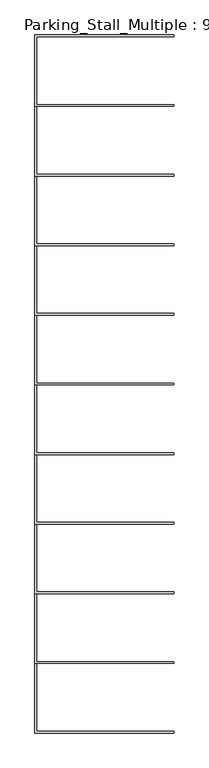
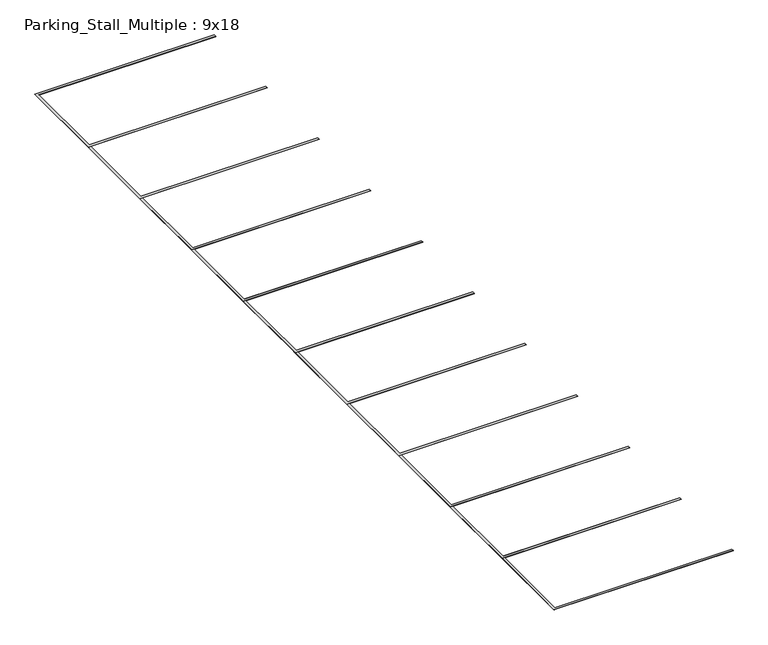
"""IFC4 building model written with IfcOpenShell, lengths in millimetres: proxy geometry, Parking_Stall_Multiple : 9x18."""

from ifc_helpers import new_model, si_unit, origin, origin_with_axes, place, context, project, spatial, polyline, outline, extrude, source, transform, mapped, element, save


def parking_stall_multiple_9x18_9482d3cf(model_context):
    return source(origin(), model_context, "Body", "SweptSolid", [
        extrude(outline(polyline([(5486.4, 24688.8), (0.0, 24688.8), (0.0, 27508.2), (5486.4, 27508.2), (5486.4, 27432.0), (76.2, 27432.0), (76.2, 24765.0), (5486.4, 24765.0), (5486.4, 24688.8)])), origin_with_axes(), (0.0, 0.0, 1.0), 6.35),
        extrude(outline(polyline([(5486.4, 21945.6), (0.0, 21945.6), (0.0, 24765.0), (5486.4, 24765.0), (5486.4, 24688.8), (76.2, 24688.8), (76.2, 22021.8), (5486.4, 22021.8), (5486.4, 21945.6)])), origin_with_axes(), (0.0, 0.0, 1.0), 6.35),
        extrude(outline(polyline([(5486.4, 19202.4), (0.0, 19202.4), (0.0, 22021.8), (5486.4, 22021.8), (5486.4, 21945.6), (76.2, 21945.6), (76.2, 19278.6), (5486.4, 19278.6), (5486.4, 19202.4)])), origin_with_axes(), (0.0, 0.0, 1.0), 6.35),
        extrude(outline(polyline([(5486.4, 16459.2), (0.0, 16459.2), (0.0, 19278.6), (5486.4, 19278.6), (5486.4, 19202.4), (76.2, 19202.4), (76.2, 16535.4), (5486.4, 16535.4), (5486.4, 16459.2)])), origin_with_axes(), (0.0, 0.0, 1.0), 6.35),
        extrude(outline(polyline([(5486.4, 13716.0), (0.0, 13716.0), (0.0, 16535.4), (5486.4, 16535.4), (5486.4, 16459.2), (76.2, 16459.2), (76.2, 13792.2), (5486.4, 13792.2), (5486.4, 13716.0)])), origin_with_axes(), (0.0, 0.0, 1.0), 6.35),
        extrude(outline(polyline([(5486.4, 10972.8), (0.0, 10972.8), (0.0, 13792.2), (5486.4, 13792.2), (5486.4, 13716.0), (76.2, 13716.0), (76.2, 11049.0), (5486.4, 11049.0), (5486.4, 10972.8)])), origin_with_axes(), (0.0, 0.0, 1.0), 6.35),
        extrude(outline(polyline([(5486.4, 8229.6), (0.0, 8229.6), (0.0, 11049.0), (5486.4, 11049.0), (5486.4, 10972.8), (76.2, 10972.8), (76.2, 8305.8), (5486.4, 8305.8), (5486.4, 8229.6)])), origin_with_axes(), (0.0, 0.0, 1.0), 6.35),
        extrude(outline(polyline([(5486.4, 5486.4), (0.0, 5486.4), (0.0, 8305.8), (5486.4, 8305.8), (5486.4, 8229.6), (76.2, 8229.6), (76.2, 5562.6), (5486.4, 5562.6), (5486.4, 5486.4)])), origin_with_axes(), (0.0, 0.0, 1.0), 6.35),
        extrude(outline(polyline([(5486.4, 2743.2), (0.0, 2743.2), (0.0, 5562.6), (5486.4, 5562.6), (5486.4, 5486.4), (76.2, 5486.4), (76.2, 2819.4), (5486.4, 2819.4), (5486.4, 2743.2)])), origin_with_axes(), (0.0, 0.0, 1.0), 6.35),
        extrude(outline(polyline([(5486.4, 0.0), (0.0, 0.0), (0.0, 2819.4), (5486.4, 2819.4), (5486.4, 2743.2), (76.2, 2743.2), (76.2, 76.2), (5486.4, 76.2), (5486.4, 0.0)])), origin_with_axes(), (0.0, 0.0, 1.0), 6.35),
    ])


if __name__ == "__main__":
    model = new_model("IFC4")
    model_context = context("Model", 3, world=origin())
    ifc_project = project(units=[si_unit("LENGTHUNIT", "METRE", prefix="MILLI")], contexts=[model_context])
    site = spatial("IfcSite", under=ifc_project)
    building = spatial("IfcBuilding", under=site)
    placement = place(None, origin())
    parking_stall_multiple_9x18_shape = parking_stall_multiple_9x18_9482d3cf(model_context)
    element("IfcBuildingElementProxy", 1, Name="Parking_Stall_Multiple : 9x18", ObjectType="Parking_Stall_Multiple : 9x18", at=placement, inside=building, context=model_context, shape_type="MappedRepresentation", body=[
        mapped(parking_stall_multiple_9x18_shape, transform((0.0, 0.0, 0.0), x_axis=(1.0, 0.0, 0.0), y_axis=(0.0, 1.0, 0.0), z_axis=(0.0, 0.0, 1.0))),
    ])
    save(model, "model.ifc")

# Revit data of these elements
# Type "Parking_Stall_Multiple : 9x18"
#   Parking_Width_M = 9' - 0"
#   Parking_Run_Length [instance default] = 65' - 0"
#   Parking_Length_M = 18' - 0"
#   Single_Parking_Visibility [instance default] = no
#   ParkingUnitsArray [instance default] = 7
#   ParkingUnits [instance default] = 7
#   Multiple_Parking_Visibility [instance default] = yes
# Element 1 (IfcBuildingElementProxy, "Parking_Stall_Multiple : 9x18")
#   Parking_Run_Length = 85' - 11.78302"
#   ParkingUnitsArray = 10
#   ParkingUnits = 10
